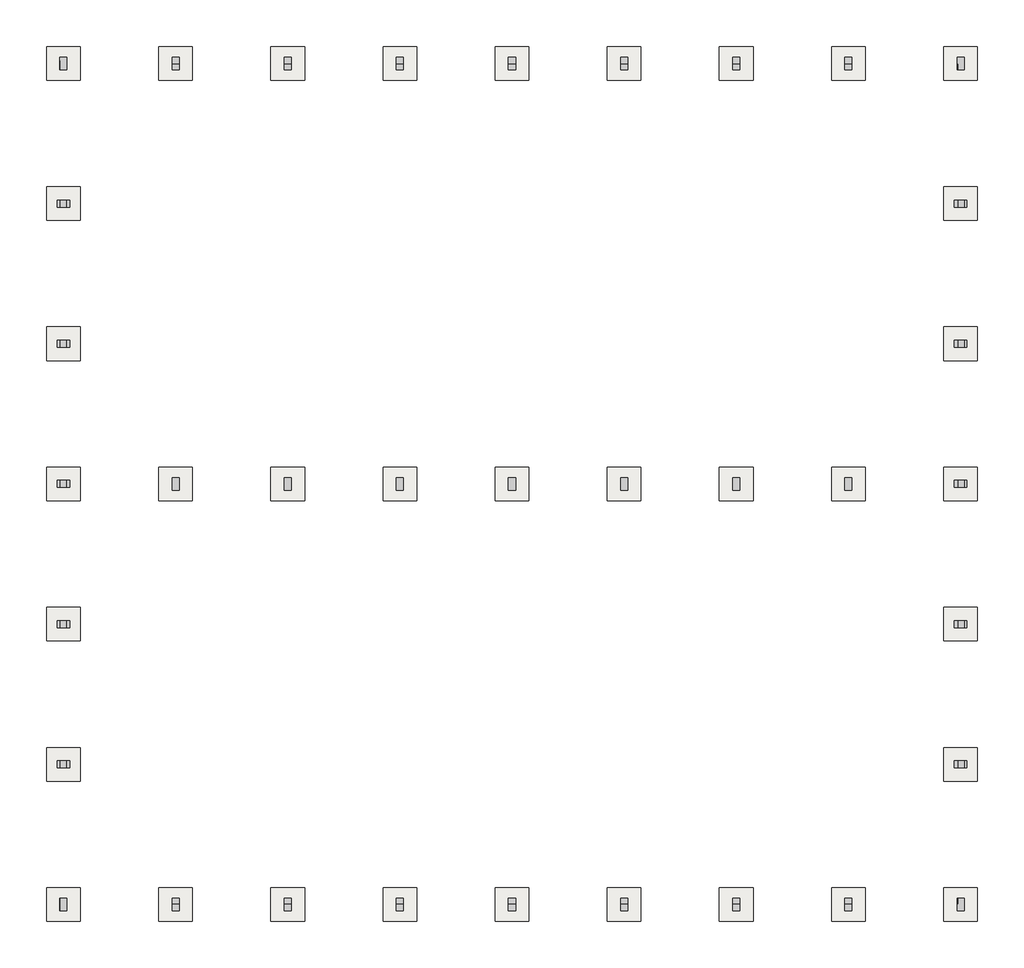
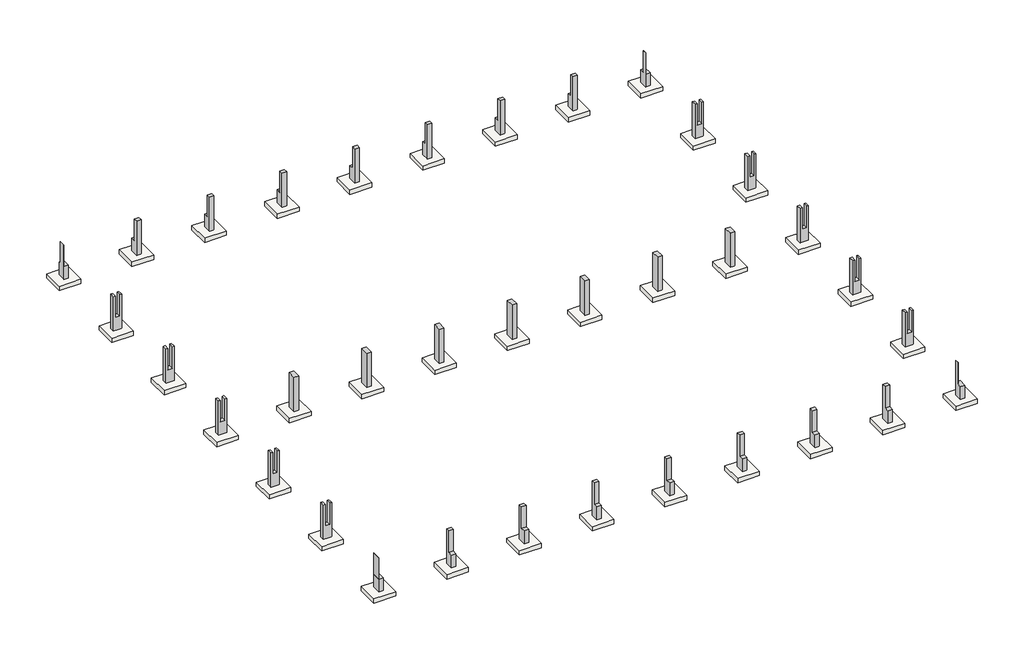
# Not in any storey: 35 columns, 35 slabs.
"""IFC4 building model written with IfcOpenShell, lengths in millimetres."""

import ifcopenshell
import ifcopenshell.guid

model = None  # the IFC model being written
_history = None  # IfcOwnerHistory: only IFC2X3 demands one
_inside = {}  # id of a spatial element -> (the spatial element, [elements in it])
_under = {}  # id of a project, library or spatial element -> (it, [spatial elements below it])
_declared = {}  # id of a project -> (the project, [libraries it declares])
_typed = {}  # id of a type object -> (the type object, [elements of that type])
_made_of = {}  # id of a material, layer set ... -> (it, [elements and type objects made of it])


def new_model(schema):
    """Start an empty IFC model of exactly this schema.

    Asked for "IFC4X3", IfcOpenShell would pick the latest addendum, in which some entities
    have other attributes; the version numbers below select the first issue.
    IFC2X3 requires an IfcOwnerHistory on every rooted entity: one is made here for all.
    """
    global model, _history
    if schema == "IFC4X3":
        model = ifcopenshell.file(schema_version=(4, 3, 0, 0))
    else:
        model = ifcopenshell.file(schema=schema)
    _inside.clear()
    _under.clear()
    _declared.clear()
    _typed.clear()
    _made_of.clear()
    _history = None
    if model.schema == "IFC2X3":
        org = make("IfcOrganization", Name="unknown")
        user = make(
            "IfcPersonAndOrganization",
            ThePerson=make("IfcPerson", FamilyName="unknown"),
            TheOrganization=org,
        )
        app = make(
            "IfcApplication",
            ApplicationDeveloper=org,
            Version="unknown",
            ApplicationFullName="unknown",
            ApplicationIdentifier="unknown",
        )
        _history = make(
            "IfcOwnerHistory",
            OwningUser=user,
            OwningApplication=app,
            ChangeAction="ADDED",
            CreationDate=0,
        )
    return model


def make(cls, **values):
    """One entity of the class cls with the attributes given. An attribute that is None is left unset."""
    return model.create_entity(
        cls, **{name: value for name, value in values.items() if value is not None}
    )


def rooted(cls, **values):
    """An entity with a GlobalId (a new one), such as an element, a storey or a relation."""
    return make(cls, GlobalId=ifcopenshell.guid.new(), OwnerHistory=_history, **values)


def si_unit(unit_type, name, prefix=None):
    """IfcSIUnit, for example si_unit("LENGTHUNIT", "METRE", prefix="MILLI")."""
    return make("IfcSIUnit", UnitType=unit_type, Prefix=prefix, Name=name)


def assignment(units):
    """IfcUnitAssignment: the units of a project."""
    return None if units is None else make("IfcUnitAssignment", Units=units)


def point(xyz):
    """IfcCartesianPoint."""
    return None if xyz is None else make("IfcCartesianPoint", Coordinates=xyz)


def direction(xyz):
    """IfcDirection."""
    return None if xyz is None else make("IfcDirection", DirectionRatios=xyz)


def frame(location, z_axis=None, x_axis=None):
    """IfcAxis2Placement3D, a coordinate frame: its origin and axes. An axis left out is left unset."""
    return make(
        "IfcAxis2Placement3D",
        Location=point(location),
        Axis=direction(z_axis),
        RefDirection=direction(x_axis),
    )


def origin():
    """The frame at (0, 0, 0) with its axes left unset."""
    return frame((0.0, 0.0, 0.0))


def place(relative_to, where):
    """IfcLocalPlacement: puts the frame where relative to a parent placement (None: the world)."""
    return make(
        "IfcLocalPlacement", PlacementRelTo=relative_to, RelativePlacement=where
    )


def context(
    kind, dimensions, precision=None, world=None, true_north=None, identifier=None
):
    """IfcGeometricRepresentationContext, for example the 3D "Model" context."""
    return make(
        "IfcGeometricRepresentationContext",
        ContextIdentifier=identifier,
        ContextType=kind,
        CoordinateSpaceDimension=dimensions,
        Precision=precision,
        WorldCoordinateSystem=world,
        TrueNorth=true_north,
    )


def project(units=None, contexts=None):
    """IfcProject with its units and contexts."""
    return rooted(
        "IfcProject",
        Name="project",
        RepresentationContexts=contexts,
        UnitsInContext=assignment(units),
    )


def spatial(cls, under=None, at=None, **own):
    """A site, building, storey or space (cls), placed at a placement, below another one or the project."""
    s = rooted(cls, ObjectPlacement=at, **own)
    if under is not None:
        _under.setdefault(under.id(), (under, []))[1].append(s)
    return s


def polyline(points):
    """IfcPolyline through the points."""
    return make("IfcPolyline", Points=[point(p) for p in points])


def outline(outer, holes=None, kind="AREA"):
    """IfcArbitraryClosedProfileDef: a profile drawn as a closed curve; with holes, ...WithVoids."""
    if holes is None:
        return make("IfcArbitraryClosedProfileDef", ProfileType=kind, OuterCurve=outer)
    return make(
        "IfcArbitraryProfileDefWithVoids",
        ProfileType=kind,
        OuterCurve=outer,
        InnerCurves=holes,
    )


def extrude(swept, where, along, depth):
    """IfcExtrudedAreaSolid: the profile swept, set in the frame where, extruded along a direction by depth."""
    return make(
        "IfcExtrudedAreaSolid",
        SweptArea=swept,
        Position=where,
        ExtrudedDirection=direction(along),
        Depth=depth,
    )


def faces_of(points, faces, orient=None, outer=None):
    """IfcFace entities. A face is a list of loops; a loop is a list of indices into points, from 0.

    orient and outer hold one flag for each loop. By default every Orientation is true, the
    first loop of a face is its IfcFaceOuterBound and the others are IfcFaceBound.
    """
    made = []
    for i, loops in enumerate(faces):
        bounds = []
        for j, loop in enumerate(loops):
            is_outer = j == 0 if outer is None else outer[i][j]
            bounds.append(
                make(
                    "IfcFaceOuterBound" if is_outer else "IfcFaceBound",
                    Bound=make("IfcPolyLoop", Polygon=[points[k] for k in loop]),
                    Orientation=True if orient is None else orient[i][j],
                )
            )
        made.append(make("IfcFace", Bounds=bounds))
    return made


def faceted_brep(points, faces, orient=None, outer=None, voids=None):
    """IfcFacetedBrep: a solid bounded by flat faces; with voids (closed shells), ...WithVoids."""
    shared = [point(p) for p in points]
    hull = make("IfcClosedShell", CfsFaces=faces_of(shared, faces, orient, outer))
    if voids is None:
        return make("IfcFacetedBrep", Outer=hull)
    return make(
        "IfcFacetedBrepWithVoids",
        Outer=hull,
        Voids=[
            make(cls, CfsFaces=faces_of(shared, fs, o, b)) for cls, fs, o, b in voids
        ],
    )


def shape(context_of_items, identifier, shape_type, items):
    """IfcShapeRepresentation: the items that make up one representation, for example the "Body"."""
    return make(
        "IfcShapeRepresentation",
        ContextOfItems=context_of_items,
        RepresentationIdentifier=identifier,
        RepresentationType=shape_type,
        Items=items,
    )


def source(mapping_origin, context_of_items, identifier, shape_type, items):
    """IfcRepresentationMap: a shape defined once, which mapped items show again and again."""
    return make(
        "IfcRepresentationMap",
        MappingOrigin=mapping_origin,
        MappedRepresentation=shape(context_of_items, identifier, shape_type, items),
    )


def transform(
    local_origin,
    x_axis=None,
    y_axis=None,
    z_axis=None,
    scale=None,
    scale2=None,
    scale3=None,
    uniform=True,
):
    """IfcCartesianTransformationOperator3D, or its non-uniform kind. x_axis, y_axis, z_axis: its Axis1, 2, 3."""
    if uniform:
        return make(
            "IfcCartesianTransformationOperator3D",
            Axis1=direction(x_axis),
            Axis2=direction(y_axis),
            LocalOrigin=point(local_origin),
            Scale=scale,
            Axis3=direction(z_axis),
        )
    return make(
        "IfcCartesianTransformationOperator3DnonUniform",
        Axis1=direction(x_axis),
        Axis2=direction(y_axis),
        LocalOrigin=point(local_origin),
        Scale=scale,
        Axis3=direction(z_axis),
        Scale2=scale2,
        Scale3=scale3,
    )


def mapped(mapping_source, mapping_target):
    """IfcMappedItem: shows the shape of a source again, moved by a transform."""
    return make(
        "IfcMappedItem", MappingSource=mapping_source, MappingTarget=mapping_target
    )


def made_of(thing, what):
    """Note that an element or type object is made of a material, layer set ...; save() writes the relation."""
    if what is not None:
        _made_of.setdefault(what.id(), (what, []))[1].append(thing)
    return thing


def element(
    cls,
    number,
    at=None,
    inside=None,
    cuts=None,
    type_object=None,
    material=None,
    context=None,
    identifier="Body",
    shape_type=None,
    held_by="IfcProductDefinitionShape",
    body=None,
    shapes=None,
    **own,
):
    """One element of the class cls, such as IfcWall. Its Tag is "e" and its number.

    at: its placement. inside: the storey or other place that contains it. cuts: it is an
    opening in that element (IfcRelVoidsElement). A single representation is given by context,
    identifier, shape_type and body (its items); several are given by shapes. held_by: the class
    of the entity that holds the representations. save() writes the other relations.
    """
    e = rooted(cls, Tag="e%d" % number, ObjectPlacement=at, **own)
    if body is not None:
        shapes = [shape(context, identifier, shape_type, body)]
    if shapes is not None:
        e.Representation = make(held_by, Representations=shapes)
    if inside is not None:
        _inside.setdefault(inside.id(), (inside, []))[1].append(e)
    if cuts is not None:
        rooted(
            "IfcRelVoidsElement", RelatingBuildingElement=cuts, RelatedOpeningElement=e
        )
    if type_object is not None:
        _typed.setdefault(type_object.id(), (type_object, []))[1].append(e)
    return made_of(e, material)


def aggregate(whole, parts):
    """IfcRelAggregates: a whole, such as a stair, and the parts it consists of."""
    return rooted("IfcRelAggregates", RelatingObject=whole, RelatedObjects=parts)


def save(model, path):
    """Write the relations noted so far, then the file.

    IfcRelAggregates (storeys below a building ...), IfcRelContainedInSpatialStructure (elements
    in a storey), IfcRelDefinesByType, IfcRelAssociatesMaterial and IfcRelDeclares: one each for
    every whole, place, type object, material and project.
    """
    for whole, parts in _under.values():
        aggregate(whole, parts)
    for where, things in _inside.values():
        rooted(
            "IfcRelContainedInSpatialStructure",
            RelatedElements=things,
            RelatingStructure=where,
        )
    for kind, things in _typed.values():
        rooted("IfcRelDefinesByType", RelatedObjects=things, RelatingType=kind)
    for what, things in _made_of.values():
        rooted("IfcRelAssociatesMaterial", RelatedObjects=things, RelatingMaterial=what)
    for by, libraries in _declared.values():
        rooted("IfcRelDeclares", RelatingContext=by, RelatedDefinitions=libraries)
    model.write(path)


def ft211_footing_rectangular_r1_5fe39465(model_context):
    return source(origin(), model_context, "Body", "SweptSolid", [
        extrude(outline(polyline([(1200.0, 1200.0), (1200.0, -1200.0), (-1200.0, -1200.0), (-1200.0, 1200.0), (1200.0, 1200.0)])), frame((0.0, 0.0, -500.0), z_axis=(0.0, 0.0, 1.0), x_axis=(1.0, 0.0, 0.0)), (0.0, 0.0, 1.0), 500.0),
    ])


model = new_model("IFC4")

# Units and contexts
model_context = context("Model", 3, world=origin())
ifc_project = project(units=[si_unit("LENGTHUNIT", "METRE", prefix="MILLI")], contexts=[model_context])

# Site, building
site = spatial("IfcSite", under=ifc_project)
building = spatial("IfcBuilding", under=site)

# Columns
placement = place(None, origin())
element("IfcColumn", 1, ObjectType="RC_Column_Rectangular : H_SC_ACC_W500xL900", at=placement, inside=building, context=model_context, shape_type="SweptSolid", body=[
    extrude(outline(polyline([(-3700.0, -450.0), (-3700.0, 450.0), (300.0, 450.0), (300.0, 254.0), (-2200.0, 254.0), (-2200.0, -246.0), (300.0, -246.0), (300.0, -450.0), (-3700.0, -450.0)])), frame((0.0, 10249.5208589, 0.0), z_axis=(0.0, 1.0, 0.0), x_axis=(0.0, 0.0, 1.0)), (0.0, 0.0, 1.0), 500.0),
])
element("IfcColumn", 2, ObjectType="RC_Column_Rectangular : H_SC_ACC_W500xL900", at=placement, inside=building, context=model_context, shape_type="SweptSolid", body=[
    extrude(outline(polyline([(-3700.0, 63550.0), (-3700.0, 64450.0), (300.0, 64450.0), (300.0, 64291.0), (-2200.0, 64291.0), (-2200.0, 63791.0), (300.0, 63791.0), (300.0, 63550.0), (-3700.0, 63550.0)])), frame((0.0, 10249.5208589, 0.0), z_axis=(0.0, 1.0, 0.0), x_axis=(0.0, 0.0, 1.0)), (0.0, 0.0, 1.0), 500.0),
])
element("IfcColumn", 3, ObjectType="RC_Column_Rectangular : H_SC_ACC_W500xL900", at=placement, inside=building, context=model_context, shape_type="Brep", body=[
    faceted_brep([(250.0, 49.5208589, -3700.0), (-250.0, 49.5208589, -3700.0), (-250.0, 949.5208589, -3700.0), (250.0, 949.5208589, -3700.0), (250.0, 49.5208589, -2200.0), (-246.0, 49.5208589, -2200.0), (-246.0, 49.5208589, 300.0), (-250.0, 49.5208589, 300.0), (-250.0, 949.5208589, 300.0), (-246.0, 949.5208589, 300.0), (-246.0, 949.5208589, -2200.0), (250.0, 949.5208589, -2200.0), (-246.0, 547.0208589, 300.0), (-246.0, 547.0208589, -2200.0)], [[[0, 1, 2, 3]], [[1, 0, 4, 5, 6, 7]], [[2, 1, 7, 8]], [[3, 2, 8, 9, 10, 11]], [[0, 3, 11, 4]], [[8, 7, 6, 12, 9]], [[6, 5, 13, 10, 9, 12]], [[10, 13, 5, 4, 11]]]),
])
element("IfcColumn", 4, ObjectType="RC_Column_Rectangular : H_SC_ACC_W500xL900", at=placement, inside=building, context=model_context, shape_type="SweptSolid", body=[
    extrude(outline(polyline([(949.5208589, -3700.0), (49.5208589, -3700.0), (49.5208589, -2200.0), (547.0208589, -2200.0), (547.0208589, 300.0), (949.5208589, 300.0), (949.5208589, -3700.0)])), frame((7750.0, 0.0, 0.0), z_axis=(1.0, 0.0, 0.0), x_axis=(0.0, 1.0, 0.0)), (0.0, 0.0, 1.0), 500.0),
])
element("IfcColumn", 5, ObjectType="RC_Column_Rectangular : H_SC_ACC_W500xL900", at=placement, inside=building, context=model_context, shape_type="SweptSolid", body=[
    extrude(outline(polyline([(949.5208589, -3700.0), (49.5208589, -3700.0), (49.5208589, -2200.0), (547.0208589, -2200.0), (547.0208589, 300.0), (949.5208589, 300.0), (949.5208589, -3700.0)])), frame((15750.0, 0.0, 0.0), z_axis=(1.0, 0.0, 0.0), x_axis=(0.0, 1.0, 0.0)), (0.0, 0.0, 1.0), 500.0),
])
element("IfcColumn", 6, ObjectType="RC_Column_Rectangular : H_SC_ACC_W500xL900", at=placement, inside=building, context=model_context, shape_type="SweptSolid", body=[
    extrude(outline(polyline([(949.5208589, -3700.0), (49.5208589, -3700.0), (49.5208589, -2200.0), (549.5208589, -2200.0), (549.5208589, 300.0), (949.5208589, 300.0), (949.5208589, -3700.0)])), frame((23750.0, 0.0, 0.0), z_axis=(1.0, 0.0, 0.0), x_axis=(0.0, 1.0, 0.0)), (0.0, 0.0, 1.0), 500.0),
])
element("IfcColumn", 7, ObjectType="RC_Column_Rectangular : H_SC_ACC_W500xL900", at=placement, inside=building, context=model_context, shape_type="SweptSolid", body=[
    extrude(outline(polyline([(949.5208589, -3700.0), (49.5208589, -3700.0), (49.5208589, -2200.0), (549.5208589, -2200.0), (549.5208589, 300.0), (949.5208589, 300.0), (949.5208589, -3700.0)])), frame((31750.0, 0.0, 0.0), z_axis=(1.0, 0.0, 0.0), x_axis=(0.0, 1.0, 0.0)), (0.0, 0.0, 1.0), 500.0),
])
element("IfcColumn", 8, ObjectType="RC_Column_Rectangular : H_SC_ACC_W500xL900", at=placement, inside=building, context=model_context, shape_type="SweptSolid", body=[
    extrude(outline(polyline([(949.5208589, -3700.0), (49.5208589, -3700.0), (49.5208589, -2200.0), (549.5208589, -2200.0), (549.5208589, 300.0), (949.5208589, 300.0), (949.5208589, -3700.0)])), frame((39750.0, 0.0, 0.0), z_axis=(1.0, 0.0, 0.0), x_axis=(0.0, 1.0, 0.0)), (0.0, 0.0, 1.0), 500.0),
])
element("IfcColumn", 9, ObjectType="RC_Column_Rectangular : H_SC_ACC_W500xL900", at=placement, inside=building, context=model_context, shape_type="SweptSolid", body=[
    extrude(outline(polyline([(949.5208589, -3700.0), (49.5208589, -3700.0), (49.5208589, -2200.0), (549.5208589, -2200.0), (549.5208589, 300.0), (949.5208589, 300.0), (949.5208589, -3700.0)])), frame((47750.0, 0.0, 0.0), z_axis=(1.0, 0.0, 0.0), x_axis=(0.0, 1.0, 0.0)), (0.0, 0.0, 1.0), 500.0),
])
element("IfcColumn", 10, ObjectType="RC_Column_Rectangular : H_SC_ACC_W500xL900", at=placement, inside=building, context=model_context, shape_type="SweptSolid", body=[
    extrude(outline(polyline([(949.5208589, -3700.0), (49.5208589, -3700.0), (49.5208589, -2200.0), (549.5208589, -2200.0), (549.5208589, 300.0), (949.5208589, 300.0), (949.5208589, -3700.0)])), frame((55750.0, 0.0, 0.0), z_axis=(1.0, 0.0, 0.0), x_axis=(0.0, 1.0, 0.0)), (0.0, 0.0, 1.0), 500.0),
])
element("IfcColumn", 11, ObjectType="RC_Column_Rectangular : H_SC_ACC_W500xL900", at=placement, inside=building, context=model_context, shape_type="Brep", body=[
    faceted_brep([(64250.0, 49.5208589, -3700.0), (63750.0, 49.5208589, -3700.0), (63750.0, 949.5208589, -3700.0), (64250.0, 949.5208589, -3700.0), (64250.0, 49.5208589, -2200.0), (63791.0, 49.5208589, -2200.0), (63750.0, 49.5208589, -2200.0), (63750.0, 549.5208589, -2200.0), (63750.0, 549.5208589, 300.0), (63750.0, 949.5208589, 300.0), (63791.0, 949.5208589, 300.0), (63791.0, 949.5208589, -2200.0), (64250.0, 949.5208589, -2200.0), (63791.0, 549.5208589, 300.0), (63791.0, 549.5208589, -2200.0)], [[[0, 1, 2, 3]], [[1, 0, 4, 5, 6]], [[2, 1, 6, 7, 8, 9]], [[3, 2, 9, 10, 11, 12]], [[0, 3, 12, 4]], [[10, 9, 8, 13]], [[11, 10, 13, 14]], [[7, 14, 13, 8]], [[4, 12, 11, 14, 7, 6, 5]]]),
])
element("IfcColumn", 12, ObjectType="RC_Column_Rectangular : H_SC_ACC_W500xL900", at=placement, inside=building, context=model_context, shape_type="SweptSolid", body=[
    extrude(outline(polyline([(-3700.0, -450.0), (-3700.0, 450.0), (300.0, 450.0), (300.0, 254.0), (-2200.0, 254.0), (-2200.0, -246.0), (300.0, -246.0), (300.0, -450.0), (-3700.0, -450.0)])), frame((0.0, 20249.5208589, 0.0), z_axis=(0.0, 1.0, 0.0), x_axis=(0.0, 0.0, 1.0)), (0.0, 0.0, 1.0), 500.0),
])
element("IfcColumn", 13, ObjectType="RC_Column_Rectangular : H_SC_ACC_W500xL900", at=placement, inside=building, context=model_context, shape_type="SweptSolid", body=[
    extrude(outline(polyline([(-3700.0, 63550.0), (-3700.0, 64450.0), (300.0, 64450.0), (300.0, 64291.0), (-2200.0, 64291.0), (-2200.0, 63791.0), (300.0, 63791.0), (300.0, 63550.0), (-3700.0, 63550.0)])), frame((0.0, 20249.5208589, 0.0), z_axis=(0.0, 1.0, 0.0), x_axis=(0.0, 0.0, 1.0)), (0.0, 0.0, 1.0), 500.0),
])
element("IfcColumn", 14, ObjectType="RC_Column_Rectangular : H_SC_ACC_W500xL900", at=placement, inside=building, context=model_context, shape_type="SweptSolid", body=[
    extrude(outline(polyline([(-3700.0, -450.0), (-3700.0, 450.0), (300.0, 450.0), (300.0, 254.0), (-2200.0, 254.0), (-2200.0, -246.0), (300.0, -246.0), (300.0, -450.0), (-3700.0, -450.0)])), frame((0.0, 30249.5208589, 0.0), z_axis=(0.0, 1.0, 0.0), x_axis=(0.0, 0.0, 1.0)), (0.0, 0.0, 1.0), 500.0),
])
element("IfcColumn", 15, ObjectType="RC_Column_Rectangular : H_SC_ACC_W500xL900", at=placement, inside=building, context=model_context, shape_type="SweptSolid", body=[
    extrude(outline(polyline([(8250.0, 30049.5208589), (7750.0, 30049.5208589), (7750.0, 30949.5208589), (8250.0, 30949.5208589), (8250.0, 30049.5208589)])), frame((0.0, 0.0, -3700.0), z_axis=(0.0, 0.0, 1.0), x_axis=(1.0, 0.0, 0.0)), (0.0, 0.0, 1.0), 4000.0),
])
element("IfcColumn", 16, ObjectType="RC_Column_Rectangular : H_SC_ACC_W500xL900", at=placement, inside=building, context=model_context, shape_type="SweptSolid", body=[
    extrude(outline(polyline([(16250.0, 30049.5208589), (15750.0, 30049.5208589), (15750.0, 30949.5208589), (16250.0, 30949.5208589), (16250.0, 30049.5208589)])), frame((0.0, 0.0, -3700.0), z_axis=(0.0, 0.0, 1.0), x_axis=(1.0, 0.0, 0.0)), (0.0, 0.0, 1.0), 4000.0),
])
element("IfcColumn", 17, ObjectType="RC_Column_Rectangular : H_SC_ACC_W500xL900", at=placement, inside=building, context=model_context, shape_type="SweptSolid", body=[
    extrude(outline(polyline([(24250.0, 30049.5208589), (23750.0, 30049.5208589), (23750.0, 30949.5208589), (24250.0, 30949.5208589), (24250.0, 30049.5208589)])), frame((0.0, 0.0, -3700.0), z_axis=(0.0, 0.0, 1.0), x_axis=(1.0, 0.0, 0.0)), (0.0, 0.0, 1.0), 4000.0),
])
element("IfcColumn", 18, ObjectType="RC_Column_Rectangular : H_SC_ACC_W500xL900", at=placement, inside=building, context=model_context, shape_type="SweptSolid", body=[
    extrude(outline(polyline([(32250.0, 30049.5208589), (31750.0, 30049.5208589), (31750.0, 30949.5208589), (32250.0, 30949.5208589), (32250.0, 30049.5208589)])), frame((0.0, 0.0, -3700.0), z_axis=(0.0, 0.0, 1.0), x_axis=(1.0, 0.0, 0.0)), (0.0, 0.0, 1.0), 4000.0),
])
element("IfcColumn", 19, ObjectType="RC_Column_Rectangular : H_SC_ACC_W500xL900", at=placement, inside=building, context=model_context, shape_type="SweptSolid", body=[
    extrude(outline(polyline([(40250.0, 30049.5208589), (39750.0, 30049.5208589), (39750.0, 30949.5208589), (40250.0, 30949.5208589), (40250.0, 30049.5208589)])), frame((0.0, 0.0, -3700.0), z_axis=(0.0, 0.0, 1.0), x_axis=(1.0, 0.0, 0.0)), (0.0, 0.0, 1.0), 4000.0),
])
element("IfcColumn", 20, ObjectType="RC_Column_Rectangular : H_SC_ACC_W500xL900", at=placement, inside=building, context=model_context, shape_type="SweptSolid", body=[
    extrude(outline(polyline([(48250.0, 30049.5208589), (47750.0, 30049.5208589), (47750.0, 30949.5208589), (48250.0, 30949.5208589), (48250.0, 30049.5208589)])), frame((0.0, 0.0, -3700.0), z_axis=(0.0, 0.0, 1.0), x_axis=(1.0, 0.0, 0.0)), (0.0, 0.0, 1.0), 4000.0),
])
element("IfcColumn", 21, ObjectType="RC_Column_Rectangular : H_SC_ACC_W500xL900", at=placement, inside=building, context=model_context, shape_type="SweptSolid", body=[
    extrude(outline(polyline([(56250.0, 30049.5208589), (55750.0, 30049.5208589), (55750.0, 30949.5208589), (56250.0, 30949.5208589), (56250.0, 30049.5208589)])), frame((0.0, 0.0, -3700.0), z_axis=(0.0, 0.0, 1.0), x_axis=(1.0, 0.0, 0.0)), (0.0, 0.0, 1.0), 4000.0),
])
element("IfcColumn", 22, ObjectType="RC_Column_Rectangular : H_SC_ACC_W500xL900", at=placement, inside=building, context=model_context, shape_type="SweptSolid", body=[
    extrude(outline(polyline([(-3700.0, 63550.0), (-3700.0, 64450.0), (300.0, 64450.0), (300.0, 64291.0), (-2200.0, 64291.0), (-2200.0, 63791.0), (300.0, 63791.0), (300.0, 63550.0), (-3700.0, 63550.0)])), frame((0.0, 30249.5208589, 0.0), z_axis=(0.0, 1.0, 0.0), x_axis=(0.0, 0.0, 1.0)), (0.0, 0.0, 1.0), 500.0),
])
element("IfcColumn", 23, ObjectType="RC_Column_Rectangular : H_SC_ACC_W500xL900", at=placement, inside=building, context=model_context, shape_type="SweptSolid", body=[
    extrude(outline(polyline([(-3700.0, -450.0), (-3700.0, 450.0), (300.0, 450.0), (300.0, 254.0), (-2200.0, 254.0), (-2200.0, -246.0), (300.0, -246.0), (300.0, -450.0), (-3700.0, -450.0)])), frame((0.0, 40249.5208589, 0.0), z_axis=(0.0, 1.0, 0.0), x_axis=(0.0, 0.0, 1.0)), (0.0, 0.0, 1.0), 500.0),
])
element("IfcColumn", 24, ObjectType="RC_Column_Rectangular : H_SC_ACC_W500xL900", at=placement, inside=building, context=model_context, shape_type="SweptSolid", body=[
    extrude(outline(polyline([(-3700.0, 63550.0), (-3700.0, 64450.0), (300.0, 64450.0), (300.0, 64291.0), (-2200.0, 64291.0), (-2200.0, 63791.0), (300.0, 63791.0), (300.0, 63550.0), (-3700.0, 63550.0)])), frame((0.0, 40249.5208589, 0.0), z_axis=(0.0, 1.0, 0.0), x_axis=(0.0, 0.0, 1.0)), (0.0, 0.0, 1.0), 500.0),
])
element("IfcColumn", 25, ObjectType="RC_Column_Rectangular : H_SC_ACC_W500xL900", at=placement, inside=building, context=model_context, shape_type="SweptSolid", body=[
    extrude(outline(polyline([(-3700.0, -450.0), (-3700.0, 450.0), (300.0, 450.0), (300.0, 254.0), (-2200.0, 254.0), (-2200.0, -246.0), (300.0, -246.0), (300.0, -450.0), (-3700.0, -450.0)])), frame((0.0, 50249.5208589, 0.0), z_axis=(0.0, 1.0, 0.0), x_axis=(0.0, 0.0, 1.0)), (0.0, 0.0, 1.0), 500.0),
])
element("IfcColumn", 26, ObjectType="RC_Column_Rectangular : H_SC_ACC_W500xL900", at=placement, inside=building, context=model_context, shape_type="SweptSolid", body=[
    extrude(outline(polyline([(-3700.0, 63550.0), (-3700.0, 64450.0), (300.0, 64450.0), (300.0, 64291.0), (-2200.0, 64291.0), (-2200.0, 63791.0), (300.0, 63791.0), (300.0, 63550.0), (-3700.0, 63550.0)])), frame((0.0, 50249.5208589, 0.0), z_axis=(0.0, 1.0, 0.0), x_axis=(0.0, 0.0, 1.0)), (0.0, 0.0, 1.0), 500.0),
])
element("IfcColumn", 27, ObjectType="RC_Column_Rectangular : H_SC_ACC_W500xL900", at=placement, inside=building, context=model_context, shape_type="Brep", body=[
    faceted_brep([(250.0, 60049.5208589, -3700.0), (-250.0, 60049.5208589, -3700.0), (-250.0, 60949.5208589, -3700.0), (250.0, 60949.5208589, -3700.0), (250.0, 60049.5208589, -2200.0), (-246.0, 60049.5208589, -2200.0), (-246.0, 60049.5208589, 300.0), (-250.0, 60049.5208589, 300.0), (-250.0, 60699.5208589, 300.0), (-250.0, 60699.5208589, -2200.0), (-250.0, 60949.5208589, -2200.0), (-217.8127408, 60949.5208589, -2200.0), (250.0, 60949.5208589, -2200.0), (-246.0, 60699.5208589, 300.0), (-246.0, 60699.5208589, -2200.0)], [[[0, 1, 2, 3]], [[1, 0, 4, 5, 6, 7]], [[2, 1, 7, 8, 9, 10]], [[3, 2, 10, 11, 12]], [[0, 3, 12, 4]], [[8, 7, 6, 13]], [[10, 9, 14, 5, 4, 12, 11]], [[9, 8, 13, 14]], [[6, 5, 14, 13]]]),
])
element("IfcColumn", 28, ObjectType="RC_Column_Rectangular : H_SC_ACC_W500xL900", at=placement, inside=building, context=model_context, shape_type="SweptSolid", body=[
    extrude(outline(polyline([(60949.5208589, -3700.0), (60049.5208589, -3700.0), (60049.5208589, 300.0), (60449.5208589, 300.0), (60449.5208589, -2200.0), (60949.5208589, -2200.0), (60949.5208589, -3700.0)])), frame((7750.0, 0.0, 0.0), z_axis=(1.0, 0.0, 0.0), x_axis=(0.0, 1.0, 0.0)), (0.0, 0.0, 1.0), 500.0),
])
element("IfcColumn", 29, ObjectType="RC_Column_Rectangular : H_SC_ACC_W500xL900", at=placement, inside=building, context=model_context, shape_type="SweptSolid", body=[
    extrude(outline(polyline([(60949.5208589, -3700.0), (60049.5208589, -3700.0), (60049.5208589, 300.0), (60449.5208589, 300.0), (60449.5208589, -2200.0), (60949.5208589, -2200.0), (60949.5208589, -3700.0)])), frame((15750.0, 0.0, 0.0), z_axis=(1.0, 0.0, 0.0), x_axis=(0.0, 1.0, 0.0)), (0.0, 0.0, 1.0), 500.0),
])
element("IfcColumn", 30, ObjectType="RC_Column_Rectangular : H_SC_ACC_W500xL900", at=placement, inside=building, context=model_context, shape_type="SweptSolid", body=[
    extrude(outline(polyline([(60949.5208589, -3700.0), (60049.5208589, -3700.0), (60049.5208589, 300.0), (60449.5208589, 300.0), (60449.5208589, -2200.0), (60949.5208589, -2200.0), (60949.5208589, -3700.0)])), frame((23750.0, 0.0, 0.0), z_axis=(1.0, 0.0, 0.0), x_axis=(0.0, 1.0, 0.0)), (0.0, 0.0, 1.0), 500.0),
])
element("IfcColumn", 31, ObjectType="RC_Column_Rectangular : H_SC_ACC_W500xL900", at=placement, inside=building, context=model_context, shape_type="SweptSolid", body=[
    extrude(outline(polyline([(60949.5208589, -3700.0), (60049.5208589, -3700.0), (60049.5208589, 300.0), (60449.5208589, 300.0), (60449.5208589, -2200.0), (60949.5208589, -2200.0), (60949.5208589, -3700.0)])), frame((31750.0, 0.0, 0.0), z_axis=(1.0, 0.0, 0.0), x_axis=(0.0, 1.0, 0.0)), (0.0, 0.0, 1.0), 500.0),
])
element("IfcColumn", 32, ObjectType="RC_Column_Rectangular : H_SC_ACC_W500xL900", at=placement, inside=building, context=model_context, shape_type="SweptSolid", body=[
    extrude(outline(polyline([(60949.5208589, -3700.0), (60049.5208589, -3700.0), (60049.5208589, 300.0), (60449.5208589, 300.0), (60449.5208589, -2200.0), (60949.5208589, -2200.0), (60949.5208589, -3700.0)])), frame((39750.0, 0.0, 0.0), z_axis=(1.0, 0.0, 0.0), x_axis=(0.0, 1.0, 0.0)), (0.0, 0.0, 1.0), 500.0),
])
element("IfcColumn", 33, ObjectType="RC_Column_Rectangular : H_SC_ACC_W500xL900", at=placement, inside=building, context=model_context, shape_type="SweptSolid", body=[
    extrude(outline(polyline([(60949.5208589, -3700.0), (60049.5208589, -3700.0), (60049.5208589, 300.0), (60449.5208589, 300.0), (60449.5208589, -2200.0), (60949.5208589, -2200.0), (60949.5208589, -3700.0)])), frame((47750.0, 0.0, 0.0), z_axis=(1.0, 0.0, 0.0), x_axis=(0.0, 1.0, 0.0)), (0.0, 0.0, 1.0), 500.0),
])
element("IfcColumn", 34, ObjectType="RC_Column_Rectangular : H_SC_ACC_W500xL900", at=placement, inside=building, context=model_context, shape_type="SweptSolid", body=[
    extrude(outline(polyline([(60949.5208589, -3700.0), (60049.5208589, -3700.0), (60049.5208589, 300.0), (60449.5208589, 300.0), (60449.5208589, -2200.0), (60949.5208589, -2200.0), (60949.5208589, -3700.0)])), frame((55750.0, 0.0, 0.0), z_axis=(1.0, 0.0, 0.0), x_axis=(0.0, 1.0, 0.0)), (0.0, 0.0, 1.0), 500.0),
])
element("IfcColumn", 35, ObjectType="RC_Column_Rectangular : H_SC_ACC_W500xL900", at=placement, inside=building, context=model_context, shape_type="Brep", body=[
    faceted_brep([(64250.0, 60049.5208589, -3700.0), (63750.0, 60049.5208589, -3700.0), (63750.0, 60949.5208589, -3700.0), (64250.0, 60949.5208589, -3700.0), (64250.0, 60049.5208589, -2200.0), (63791.0, 60049.5208589, -2200.0), (63791.0, 60049.5208589, 300.0), (63750.0, 60049.5208589, 300.0), (63750.0, 60449.5208589, 300.0), (63750.0, 60449.5208589, -2200.0), (63750.0, 60949.5208589, -2200.0), (64250.0, 60949.5208589, -2200.0), (63791.0, 60449.5208589, 300.0), (63791.0, 60449.5208589, -2200.0)], [[[0, 1, 2, 3]], [[1, 0, 4, 5, 6, 7]], [[2, 1, 7, 8, 9, 10]], [[3, 2, 10, 11]], [[0, 3, 11, 4]], [[8, 7, 6, 12]], [[9, 8, 12, 13]], [[5, 13, 12, 6]], [[10, 9, 13, 5, 4, 11]]]),
])

# Slabs
ft211_footing_rectangular_r1_shape = ft211_footing_rectangular_r1_5fe39465(model_context)
element("IfcSlab", 36, ObjectType="FT211-Footing-Rectangular_R1 : H_SF_ACF_W2400xL2400xT500_Bitumen", at=placement, inside=building, context=model_context, shape_type="MappedRepresentation", body=[
    mapped(ft211_footing_rectangular_r1_shape, transform((0.0, 10499.5208589, -3700.0), x_axis=(1.0, 0.0, 0.0), y_axis=(0.0, 1.0, 0.0), z_axis=(0.0, 0.0, 1.0))),
])
element("IfcSlab", 37, ObjectType="FT211-Footing-Rectangular_R1 : H_SF_ACF_W2400xL2400xT500_Bitumen", at=placement, inside=building, context=model_context, shape_type="MappedRepresentation", body=[
    mapped(ft211_footing_rectangular_r1_shape, transform((64000.0, 10499.5208589, -3700.0), x_axis=(1.0, 0.0, 0.0), y_axis=(0.0, 1.0, 0.0), z_axis=(0.0, 0.0, 1.0))),
])
element("IfcSlab", 38, ObjectType="FT211-Footing-Rectangular_R1 : H_SF_ACF_W2400xL2400xT500_Bitumen", at=placement, inside=building, context=model_context, shape_type="MappedRepresentation", body=[
    mapped(ft211_footing_rectangular_r1_shape, transform((0.0, 499.5208589, -3700.0), x_axis=(1.0, 0.0, 0.0), y_axis=(0.0, 1.0, 0.0), z_axis=(0.0, 0.0, 1.0))),
])
element("IfcSlab", 39, ObjectType="FT211-Footing-Rectangular_R1 : H_SF_ACF_W2400xL2400xT500_Bitumen", at=placement, inside=building, context=model_context, shape_type="MappedRepresentation", body=[
    mapped(ft211_footing_rectangular_r1_shape, transform((8000.0, 499.5208589, -3700.0), x_axis=(1.0, 0.0, 0.0), y_axis=(0.0, 1.0, 0.0), z_axis=(0.0, 0.0, 1.0))),
])
element("IfcSlab", 40, ObjectType="FT211-Footing-Rectangular_R1 : H_SF_ACF_W2400xL2400xT500_Bitumen", at=placement, inside=building, context=model_context, shape_type="MappedRepresentation", body=[
    mapped(ft211_footing_rectangular_r1_shape, transform((16000.0, 499.5208589, -3700.0), x_axis=(1.0, 0.0, 0.0), y_axis=(0.0, 1.0, 0.0), z_axis=(0.0, 0.0, 1.0))),
])
element("IfcSlab", 41, ObjectType="FT211-Footing-Rectangular_R1 : H_SF_ACF_W2400xL2400xT500_Bitumen", at=placement, inside=building, context=model_context, shape_type="MappedRepresentation", body=[
    mapped(ft211_footing_rectangular_r1_shape, transform((24000.0, 499.5208589, -3700.0), x_axis=(1.0, 0.0, 0.0), y_axis=(0.0, 1.0, 0.0), z_axis=(0.0, 0.0, 1.0))),
])
element("IfcSlab", 42, ObjectType="FT211-Footing-Rectangular_R1 : H_SF_ACF_W2400xL2400xT500_Bitumen", at=placement, inside=building, context=model_context, shape_type="MappedRepresentation", body=[
    mapped(ft211_footing_rectangular_r1_shape, transform((32000.0, 499.5208589, -3700.0), x_axis=(1.0, 0.0, 0.0), y_axis=(0.0, 1.0, 0.0), z_axis=(0.0, 0.0, 1.0))),
])
element("IfcSlab", 43, ObjectType="FT211-Footing-Rectangular_R1 : H_SF_ACF_W2400xL2400xT500_Bitumen", at=placement, inside=building, context=model_context, shape_type="MappedRepresentation", body=[
    mapped(ft211_footing_rectangular_r1_shape, transform((40000.0, 499.5208589, -3700.0), x_axis=(1.0, 0.0, 0.0), y_axis=(0.0, 1.0, 0.0), z_axis=(0.0, 0.0, 1.0))),
])
element("IfcSlab", 44, ObjectType="FT211-Footing-Rectangular_R1 : H_SF_ACF_W2400xL2400xT500_Bitumen", at=placement, inside=building, context=model_context, shape_type="MappedRepresentation", body=[
    mapped(ft211_footing_rectangular_r1_shape, transform((48000.0, 499.5208589, -3700.0), x_axis=(1.0, 0.0, 0.0), y_axis=(0.0, 1.0, 0.0), z_axis=(0.0, 0.0, 1.0))),
])
element("IfcSlab", 45, ObjectType="FT211-Footing-Rectangular_R1 : H_SF_ACF_W2400xL2400xT500_Bitumen", at=placement, inside=building, context=model_context, shape_type="MappedRepresentation", body=[
    mapped(ft211_footing_rectangular_r1_shape, transform((56000.0, 499.5208589, -3700.0), x_axis=(1.0, 0.0, 0.0), y_axis=(0.0, 1.0, 0.0), z_axis=(0.0, 0.0, 1.0))),
])
element("IfcSlab", 46, ObjectType="FT211-Footing-Rectangular_R1 : H_SF_ACF_W2400xL2400xT500_Bitumen", at=placement, inside=building, context=model_context, shape_type="MappedRepresentation", body=[
    mapped(ft211_footing_rectangular_r1_shape, transform((64000.0, 499.5208589, -3700.0), x_axis=(1.0, 0.0, 0.0), y_axis=(0.0, 1.0, 0.0), z_axis=(0.0, 0.0, 1.0))),
])
element("IfcSlab", 47, ObjectType="FT211-Footing-Rectangular_R1 : H_SF_ACF_W2400xL2400xT500_Bitumen", at=placement, inside=building, context=model_context, shape_type="MappedRepresentation", body=[
    mapped(ft211_footing_rectangular_r1_shape, transform((0.0, 20499.5208589, -3700.0), x_axis=(1.0, 0.0, 0.0), y_axis=(0.0, 1.0, 0.0), z_axis=(0.0, 0.0, 1.0))),
])
element("IfcSlab", 48, ObjectType="FT211-Footing-Rectangular_R1 : H_SF_ACF_W2400xL2400xT500_Bitumen", at=placement, inside=building, context=model_context, shape_type="MappedRepresentation", body=[
    mapped(ft211_footing_rectangular_r1_shape, transform((64000.0, 20499.5208589, -3700.0), x_axis=(1.0, 0.0, 0.0), y_axis=(0.0, 1.0, 0.0), z_axis=(0.0, 0.0, 1.0))),
])
element("IfcSlab", 49, ObjectType="FT211-Footing-Rectangular_R1 : H_SF_ACF_W2400xL2400xT500_Bitumen", at=placement, inside=building, context=model_context, shape_type="MappedRepresentation", body=[
    mapped(ft211_footing_rectangular_r1_shape, transform((0.0, 30499.5208589, -3700.0), x_axis=(1.0, 0.0, 0.0), y_axis=(0.0, 1.0, 0.0), z_axis=(0.0, 0.0, 1.0))),
])
element("IfcSlab", 50, ObjectType="FT211-Footing-Rectangular_R1 : H_SF_ACF_W2400xL2400xT500_Bitumen", at=placement, inside=building, context=model_context, shape_type="MappedRepresentation", body=[
    mapped(ft211_footing_rectangular_r1_shape, transform((8000.0, 30499.5208589, -3700.0), x_axis=(1.0, 0.0, 0.0), y_axis=(0.0, 1.0, 0.0), z_axis=(0.0, 0.0, 1.0))),
])
element("IfcSlab", 51, ObjectType="FT211-Footing-Rectangular_R1 : H_SF_ACF_W2400xL2400xT500_Bitumen", at=placement, inside=building, context=model_context, shape_type="MappedRepresentation", body=[
    mapped(ft211_footing_rectangular_r1_shape, transform((16000.0, 30499.5208589, -3700.0), x_axis=(1.0, 0.0, 0.0), y_axis=(0.0, 1.0, 0.0), z_axis=(0.0, 0.0, 1.0))),
])
element("IfcSlab", 52, ObjectType="FT211-Footing-Rectangular_R1 : H_SF_ACF_W2400xL2400xT500_Bitumen", at=placement, inside=building, context=model_context, shape_type="MappedRepresentation", body=[
    mapped(ft211_footing_rectangular_r1_shape, transform((24000.0, 30499.5208589, -3700.0), x_axis=(1.0, 0.0, 0.0), y_axis=(0.0, 1.0, 0.0), z_axis=(0.0, 0.0, 1.0))),
])
element("IfcSlab", 53, ObjectType="FT211-Footing-Rectangular_R1 : H_SF_ACF_W2400xL2400xT500_Bitumen", at=placement, inside=building, context=model_context, shape_type="MappedRepresentation", body=[
    mapped(ft211_footing_rectangular_r1_shape, transform((32000.0, 30499.5208589, -3700.0), x_axis=(1.0, 0.0, 0.0), y_axis=(0.0, 1.0, 0.0), z_axis=(0.0, 0.0, 1.0))),
])
element("IfcSlab", 54, ObjectType="FT211-Footing-Rectangular_R1 : H_SF_ACF_W2400xL2400xT500_Bitumen", at=placement, inside=building, context=model_context, shape_type="MappedRepresentation", body=[
    mapped(ft211_footing_rectangular_r1_shape, transform((40000.0, 30499.5208589, -3700.0), x_axis=(1.0, 0.0, 0.0), y_axis=(0.0, 1.0, 0.0), z_axis=(0.0, 0.0, 1.0))),
])
element("IfcSlab", 55, ObjectType="FT211-Footing-Rectangular_R1 : H_SF_ACF_W2400xL2400xT500_Bitumen", at=placement, inside=building, context=model_context, shape_type="MappedRepresentation", body=[
    mapped(ft211_footing_rectangular_r1_shape, transform((48000.0, 30499.5208589, -3700.0), x_axis=(1.0, 0.0, 0.0), y_axis=(0.0, 1.0, 0.0), z_axis=(0.0, 0.0, 1.0))),
])
element("IfcSlab", 56, ObjectType="FT211-Footing-Rectangular_R1 : H_SF_ACF_W2400xL2400xT500_Bitumen", at=placement, inside=building, context=model_context, shape_type="MappedRepresentation", body=[
    mapped(ft211_footing_rectangular_r1_shape, transform((56000.0, 30499.5208589, -3700.0), x_axis=(1.0, 0.0, 0.0), y_axis=(0.0, 1.0, 0.0), z_axis=(0.0, 0.0, 1.0))),
])
element("IfcSlab", 57, ObjectType="FT211-Footing-Rectangular_R1 : H_SF_ACF_W2400xL2400xT500_Bitumen", at=placement, inside=building, context=model_context, shape_type="MappedRepresentation", body=[
    mapped(ft211_footing_rectangular_r1_shape, transform((64000.0, 30499.5208589, -3700.0), x_axis=(1.0, 0.0, 0.0), y_axis=(0.0, 1.0, 0.0), z_axis=(0.0, 0.0, 1.0))),
])
element("IfcSlab", 58, ObjectType="FT211-Footing-Rectangular_R1 : H_SF_ACF_W2400xL2400xT500_Bitumen", at=placement, inside=building, context=model_context, shape_type="MappedRepresentation", body=[
    mapped(ft211_footing_rectangular_r1_shape, transform((0.0, 40499.5208589, -3700.0), x_axis=(1.0, 0.0, 0.0), y_axis=(0.0, 1.0, 0.0), z_axis=(0.0, 0.0, 1.0))),
])
element("IfcSlab", 59, ObjectType="FT211-Footing-Rectangular_R1 : H_SF_ACF_W2400xL2400xT500_Bitumen", at=placement, inside=building, context=model_context, shape_type="MappedRepresentation", body=[
    mapped(ft211_footing_rectangular_r1_shape, transform((64000.0, 40499.5208589, -3700.0), x_axis=(1.0, 0.0, 0.0), y_axis=(0.0, 1.0, 0.0), z_axis=(0.0, 0.0, 1.0))),
])
element("IfcSlab", 60, ObjectType="FT211-Footing-Rectangular_R1 : H_SF_ACF_W2400xL2400xT500_Bitumen", at=placement, inside=building, context=model_context, shape_type="MappedRepresentation", body=[
    mapped(ft211_footing_rectangular_r1_shape, transform((0.0, 50499.5208589, -3700.0), x_axis=(1.0, 0.0, 0.0), y_axis=(0.0, 1.0, 0.0), z_axis=(0.0, 0.0, 1.0))),
])
element("IfcSlab", 61, ObjectType="FT211-Footing-Rectangular_R1 : H_SF_ACF_W2400xL2400xT500_Bitumen", at=placement, inside=building, context=model_context, shape_type="MappedRepresentation", body=[
    mapped(ft211_footing_rectangular_r1_shape, transform((64000.0, 50499.5208589, -3700.0), x_axis=(1.0, 0.0, 0.0), y_axis=(0.0, 1.0, 0.0), z_axis=(0.0, 0.0, 1.0))),
])
element("IfcSlab", 62, ObjectType="FT211-Footing-Rectangular_R1 : H_SF_ACF_W2400xL2400xT500_Bitumen", at=placement, inside=building, context=model_context, shape_type="MappedRepresentation", body=[
    mapped(ft211_footing_rectangular_r1_shape, transform((0.0, 60499.5208589, -3700.0), x_axis=(1.0, 0.0, 0.0), y_axis=(0.0, 1.0, 0.0), z_axis=(0.0, 0.0, 1.0))),
])
element("IfcSlab", 63, ObjectType="FT211-Footing-Rectangular_R1 : H_SF_ACF_W2400xL2400xT500_Bitumen", at=placement, inside=building, context=model_context, shape_type="MappedRepresentation", body=[
    mapped(ft211_footing_rectangular_r1_shape, transform((8000.0, 60499.5208589, -3700.0), x_axis=(1.0, 0.0, 0.0), y_axis=(0.0, 1.0, 0.0), z_axis=(0.0, 0.0, 1.0))),
])
element("IfcSlab", 64, ObjectType="FT211-Footing-Rectangular_R1 : H_SF_ACF_W2400xL2400xT500_Bitumen", at=placement, inside=building, context=model_context, shape_type="MappedRepresentation", body=[
    mapped(ft211_footing_rectangular_r1_shape, transform((16000.0, 60499.5208589, -3700.0), x_axis=(1.0, 0.0, 0.0), y_axis=(0.0, 1.0, 0.0), z_axis=(0.0, 0.0, 1.0))),
])
element("IfcSlab", 65, ObjectType="FT211-Footing-Rectangular_R1 : H_SF_ACF_W2400xL2400xT500_Bitumen", at=placement, inside=building, context=model_context, shape_type="MappedRepresentation", body=[
    mapped(ft211_footing_rectangular_r1_shape, transform((24000.0, 60499.5208589, -3700.0), x_axis=(1.0, 0.0, 0.0), y_axis=(0.0, 1.0, 0.0), z_axis=(0.0, 0.0, 1.0))),
])
element("IfcSlab", 66, ObjectType="FT211-Footing-Rectangular_R1 : H_SF_ACF_W2400xL2400xT500_Bitumen", at=placement, inside=building, context=model_context, shape_type="MappedRepresentation", body=[
    mapped(ft211_footing_rectangular_r1_shape, transform((32000.0, 60499.5208589, -3700.0), x_axis=(1.0, 0.0, 0.0), y_axis=(0.0, 1.0, 0.0), z_axis=(0.0, 0.0, 1.0))),
])
element("IfcSlab", 67, ObjectType="FT211-Footing-Rectangular_R1 : H_SF_ACF_W2400xL2400xT500_Bitumen", at=placement, inside=building, context=model_context, shape_type="MappedRepresentation", body=[
    mapped(ft211_footing_rectangular_r1_shape, transform((40000.0, 60499.5208589, -3700.0), x_axis=(1.0, 0.0, 0.0), y_axis=(0.0, 1.0, 0.0), z_axis=(0.0, 0.0, 1.0))),
])
element("IfcSlab", 68, ObjectType="FT211-Footing-Rectangular_R1 : H_SF_ACF_W2400xL2400xT500_Bitumen", at=placement, inside=building, context=model_context, shape_type="MappedRepresentation", body=[
    mapped(ft211_footing_rectangular_r1_shape, transform((48000.0, 60499.5208589, -3700.0), x_axis=(1.0, 0.0, 0.0), y_axis=(0.0, 1.0, 0.0), z_axis=(0.0, 0.0, 1.0))),
])
element("IfcSlab", 69, ObjectType="FT211-Footing-Rectangular_R1 : H_SF_ACF_W2400xL2400xT500_Bitumen", at=placement, inside=building, context=model_context, shape_type="MappedRepresentation", body=[
    mapped(ft211_footing_rectangular_r1_shape, transform((56000.0, 60499.5208589, -3700.0), x_axis=(1.0, 0.0, 0.0), y_axis=(0.0, 1.0, 0.0), z_axis=(0.0, 0.0, 1.0))),
])
element("IfcSlab", 70, ObjectType="FT211-Footing-Rectangular_R1 : H_SF_ACF_W2400xL2400xT500_Bitumen", at=placement, inside=building, context=model_context, shape_type="MappedRepresentation", body=[
    mapped(ft211_footing_rectangular_r1_shape, transform((64000.0, 60499.5208589, -3700.0), x_axis=(1.0, 0.0, 0.0), y_axis=(0.0, 1.0, 0.0), z_axis=(0.0, 0.0, 1.0))),
])

save(model, "model.ifc")

# Revit data of these elements
# Type "RC_Column_Rectangular : H_SC_ACC_W500xL900"
#   Width = 900 mm
#   Length = 500 mm
#   hec_material3 [instance default] = none
#   hec_material2 [instance default] = none
#   hec_material1 [instance default] = none
#   Structural Material [instance default] = none
#   Description = (empty or 0)
# Type "FT211-Footing-Rectangular_R1 : H_SF_ACF_W2400xL2400xT500_Bitumen"
#   Top bar = "D25@300"
#   Description = "UG Shallow Foundation"
#   Bottom bar = "D20@300"
#   Width = 2400 mm
#   Length = 2400 mm
#   Foundation Thickness = 500 mm
#   Structural Material [instance default] = none
#   Assembly Code = ""
# Elements 1, 2, 3, 4, 5, 6, 7, 8, 9, 10, 11, 12, 13, 14, 15, 16, 17, 18, 19, 20, 21, 22, 23, 24, 25, 26, 27, 28, 29, 30, 31, 32, 33, 34, 35 (IfcColumn, "RC_Column_Rectangular : H_SC_ACC_W500xL900")
#   Comments = ""
#   hec_material3 = none
#   hec_material2 = none
#   hec_material1 = none
#   Structural Material = none
#   Phase Created = New Construction
# Elements 36, 37, 38, 39, 40, 41, 42, 43, 44, 45, 46, 47, 48, 49, 50, 51, 52, 53, 54, 55, 56, 57, 58, 59, 60, 61, 62, 63, 64, 65, 66, 67, 68, 69, 70 (IfcSlab, "FT211-Footing-Rectangular_R1 : H_SF_ACF_W2400xL2400xT500_Bitumen")
#   Comments = ""
#   Structural Material = none
#   Phase Created = New Construction
